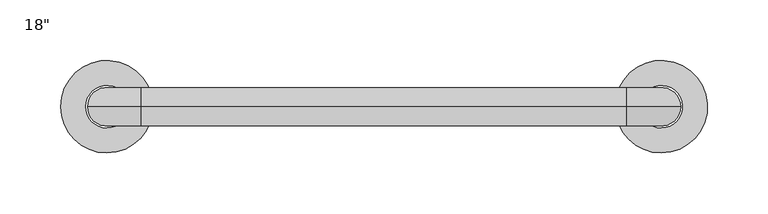
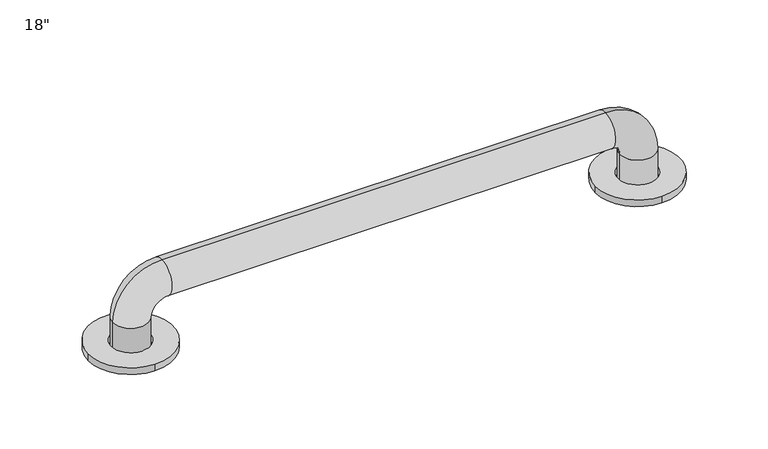
"""IFC4 building model written with IfcOpenShell, lengths in millimetres: proxy geometry."""

import ifcopenshell
import ifcopenshell.guid

model = None  # the IFC model being written
_history = None  # IfcOwnerHistory: only IFC2X3 demands one
_inside = {}  # id of a spatial element -> (the spatial element, [elements in it])
_under = {}  # id of a project, library or spatial element -> (it, [spatial elements below it])
_declared = {}  # id of a project -> (the project, [libraries it declares])
_typed = {}  # id of a type object -> (the type object, [elements of that type])
_made_of = {}  # id of a material, layer set ... -> (it, [elements and type objects made of it])


def new_model(schema):
    """Start an empty IFC model of exactly this schema.

    Asked for "IFC4X3", IfcOpenShell would pick the latest addendum, in which some entities
    have other attributes; the version numbers below select the first issue.
    IFC2X3 requires an IfcOwnerHistory on every rooted entity: one is made here for all.
    """
    global model, _history
    if schema == "IFC4X3":
        model = ifcopenshell.file(schema_version=(4, 3, 0, 0))
    else:
        model = ifcopenshell.file(schema=schema)
    _inside.clear()
    _under.clear()
    _declared.clear()
    _typed.clear()
    _made_of.clear()
    _history = None
    if model.schema == "IFC2X3":
        org = make("IfcOrganization", Name="unknown")
        user = make(
            "IfcPersonAndOrganization",
            ThePerson=make("IfcPerson", FamilyName="unknown"),
            TheOrganization=org,
        )
        app = make(
            "IfcApplication",
            ApplicationDeveloper=org,
            Version="unknown",
            ApplicationFullName="unknown",
            ApplicationIdentifier="unknown",
        )
        _history = make(
            "IfcOwnerHistory",
            OwningUser=user,
            OwningApplication=app,
            ChangeAction="ADDED",
            CreationDate=0,
        )
    return model


def make(cls, **values):
    """One entity of the class cls with the attributes given. An attribute that is None is left unset."""
    return model.create_entity(
        cls, **{name: value for name, value in values.items() if value is not None}
    )


def rooted(cls, **values):
    """An entity with a GlobalId (a new one), such as an element, a storey or a relation."""
    return make(cls, GlobalId=ifcopenshell.guid.new(), OwnerHistory=_history, **values)


def si_unit(unit_type, name, prefix=None):
    """IfcSIUnit, for example si_unit("LENGTHUNIT", "METRE", prefix="MILLI")."""
    return make("IfcSIUnit", UnitType=unit_type, Prefix=prefix, Name=name)


def assignment(units):
    """IfcUnitAssignment: the units of a project."""
    return None if units is None else make("IfcUnitAssignment", Units=units)


def point(xyz):
    """IfcCartesianPoint."""
    return None if xyz is None else make("IfcCartesianPoint", Coordinates=xyz)


def direction(xyz):
    """IfcDirection."""
    return None if xyz is None else make("IfcDirection", DirectionRatios=xyz)


def frame(location, z_axis=None, x_axis=None):
    """IfcAxis2Placement3D, a coordinate frame: its origin and axes. An axis left out is left unset."""
    return make(
        "IfcAxis2Placement3D",
        Location=point(location),
        Axis=direction(z_axis),
        RefDirection=direction(x_axis),
    )


def frame_2d(location, x_axis=None):
    """IfcAxis2Placement2D, a coordinate frame in the plane: its origin and x axis."""
    return make(
        "IfcAxis2Placement2D", Location=point(location), RefDirection=direction(x_axis)
    )


def origin():
    """The frame at (0, 0, 0) with its axes left unset."""
    return frame((0.0, 0.0, 0.0))


def origin_with_axes():
    """The frame at (0, 0, 0) with the z axis (0, 0, 1) and the x axis (1, 0, 0) written out."""
    return frame((0.0, 0.0, 0.0), z_axis=(0.0, 0.0, 1.0), x_axis=(1.0, 0.0, 0.0))


def origin_2d():
    """The frame at (0, 0) in the plane with its x axis left unset."""
    return frame_2d((0.0, 0.0))


def place(relative_to, where):
    """IfcLocalPlacement: puts the frame where relative to a parent placement (None: the world)."""
    return make(
        "IfcLocalPlacement", PlacementRelTo=relative_to, RelativePlacement=where
    )


def context(
    kind, dimensions, precision=None, world=None, true_north=None, identifier=None
):
    """IfcGeometricRepresentationContext, for example the 3D "Model" context."""
    return make(
        "IfcGeometricRepresentationContext",
        ContextIdentifier=identifier,
        ContextType=kind,
        CoordinateSpaceDimension=dimensions,
        Precision=precision,
        WorldCoordinateSystem=world,
        TrueNorth=true_north,
    )


def project(units=None, contexts=None):
    """IfcProject with its units and contexts."""
    return rooted(
        "IfcProject",
        Name="project",
        RepresentationContexts=contexts,
        UnitsInContext=assignment(units),
    )


def spatial(cls, under=None, at=None, **own):
    """A site, building, storey or space (cls), placed at a placement, below another one or the project."""
    s = rooted(cls, ObjectPlacement=at, **own)
    if under is not None:
        _under.setdefault(under.id(), (under, []))[1].append(s)
    return s


def circle_curve(where, radius):
    """IfcCircle in the frame where."""
    return make("IfcCircle", Position=where, Radius=radius)


def ellipse_curve(where, semi_axis1, semi_axis2):
    """IfcEllipse in the frame where."""
    return make(
        "IfcEllipse", Position=where, SemiAxis1=semi_axis1, SemiAxis2=semi_axis2
    )


def trimmed(basis, trim1, trim2, sense, master):
    """IfcTrimmedCurve: the piece of a basis curve between two trims."""
    return make(
        "IfcTrimmedCurve",
        BasisCurve=basis,
        Trim1=trim1,
        Trim2=trim2,
        SenseAgreement=sense,
        MasterRepresentation=master,
    )


def segment(curve, same_sense, transition):
    """IfcCompositeCurveSegment."""
    return make(
        "IfcCompositeCurveSegment",
        Transition=transition,
        SameSense=same_sense,
        ParentCurve=curve,
    )


def composite_curve(segments, self_intersect=None):
    """IfcCompositeCurve: segments joined end to end."""
    return make("IfcCompositeCurve", Segments=segments, SelfIntersect=self_intersect)


def outline(outer, holes=None, kind="AREA"):
    """IfcArbitraryClosedProfileDef: a profile drawn as a closed curve; with holes, ...WithVoids."""
    if holes is None:
        return make("IfcArbitraryClosedProfileDef", ProfileType=kind, OuterCurve=outer)
    return make(
        "IfcArbitraryProfileDefWithVoids",
        ProfileType=kind,
        OuterCurve=outer,
        InnerCurves=holes,
    )


def extrude(swept, where, along, depth):
    """IfcExtrudedAreaSolid: the profile swept, set in the frame where, extruded along a direction by depth."""
    return make(
        "IfcExtrudedAreaSolid",
        SweptArea=swept,
        Position=where,
        ExtrudedDirection=direction(along),
        Depth=depth,
    )


def shape(context_of_items, identifier, shape_type, items):
    """IfcShapeRepresentation: the items that make up one representation, for example the "Body"."""
    return make(
        "IfcShapeRepresentation",
        ContextOfItems=context_of_items,
        RepresentationIdentifier=identifier,
        RepresentationType=shape_type,
        Items=items,
    )


def source(mapping_origin, context_of_items, identifier, shape_type, items):
    """IfcRepresentationMap: a shape defined once, which mapped items show again and again."""
    return make(
        "IfcRepresentationMap",
        MappingOrigin=mapping_origin,
        MappedRepresentation=shape(context_of_items, identifier, shape_type, items),
    )


def transform(
    local_origin,
    x_axis=None,
    y_axis=None,
    z_axis=None,
    scale=None,
    scale2=None,
    scale3=None,
    uniform=True,
):
    """IfcCartesianTransformationOperator3D, or its non-uniform kind. x_axis, y_axis, z_axis: its Axis1, 2, 3."""
    if uniform:
        return make(
            "IfcCartesianTransformationOperator3D",
            Axis1=direction(x_axis),
            Axis2=direction(y_axis),
            LocalOrigin=point(local_origin),
            Scale=scale,
            Axis3=direction(z_axis),
        )
    return make(
        "IfcCartesianTransformationOperator3DnonUniform",
        Axis1=direction(x_axis),
        Axis2=direction(y_axis),
        LocalOrigin=point(local_origin),
        Scale=scale,
        Axis3=direction(z_axis),
        Scale2=scale2,
        Scale3=scale3,
    )


def mapped(mapping_source, mapping_target):
    """IfcMappedItem: shows the shape of a source again, moved by a transform."""
    return make(
        "IfcMappedItem", MappingSource=mapping_source, MappingTarget=mapping_target
    )


def made_of(thing, what):
    """Note that an element or type object is made of a material, layer set ...; save() writes the relation."""
    if what is not None:
        _made_of.setdefault(what.id(), (what, []))[1].append(thing)
    return thing


def element(
    cls,
    number,
    at=None,
    inside=None,
    cuts=None,
    type_object=None,
    material=None,
    context=None,
    identifier="Body",
    shape_type=None,
    held_by="IfcProductDefinitionShape",
    body=None,
    shapes=None,
    **own,
):
    """One element of the class cls, such as IfcWall. Its Tag is "e" and its number.

    at: its placement. inside: the storey or other place that contains it. cuts: it is an
    opening in that element (IfcRelVoidsElement). A single representation is given by context,
    identifier, shape_type and body (its items); several are given by shapes. held_by: the class
    of the entity that holds the representations. save() writes the other relations.
    """
    e = rooted(cls, Tag="e%d" % number, ObjectPlacement=at, **own)
    if body is not None:
        shapes = [shape(context, identifier, shape_type, body)]
    if shapes is not None:
        e.Representation = make(held_by, Representations=shapes)
    if inside is not None:
        _inside.setdefault(inside.id(), (inside, []))[1].append(e)
    if cuts is not None:
        rooted(
            "IfcRelVoidsElement", RelatingBuildingElement=cuts, RelatedOpeningElement=e
        )
    if type_object is not None:
        _typed.setdefault(type_object.id(), (type_object, []))[1].append(e)
    return made_of(e, material)


def aggregate(whole, parts):
    """IfcRelAggregates: a whole, such as a stair, and the parts it consists of."""
    return rooted("IfcRelAggregates", RelatingObject=whole, RelatedObjects=parts)


def save(model, path):
    """Write the relations noted so far, then the file.

    IfcRelAggregates (storeys below a building ...), IfcRelContainedInSpatialStructure (elements
    in a storey), IfcRelDefinesByType, IfcRelAssociatesMaterial and IfcRelDeclares: one each for
    every whole, place, type object, material and project.
    """
    for whole, parts in _under.values():
        aggregate(whole, parts)
    for where, things in _inside.values():
        rooted(
            "IfcRelContainedInSpatialStructure",
            RelatedElements=things,
            RelatingStructure=where,
        )
    for kind, things in _typed.values():
        rooted("IfcRelDefinesByType", RelatedObjects=things, RelatingType=kind)
    for what, things in _made_of.values():
        rooted("IfcRelAssociatesMaterial", RelatedObjects=things, RelatingMaterial=what)
    for by, libraries in _declared.values():
        rooted("IfcRelDeclares", RelatingContext=by, RelatedDefinitions=libraries)
    model.write(path)


def plane_surface(at):
    """IfcPlane: the flat surface through the origin of the frame at, square to its z axis."""
    return make("IfcPlane", Position=at)


def cylinder_surface(at, radius):
    """IfcCylindricalSurface: all points at the distance radius from the z axis of the frame at."""
    return make("IfcCylindricalSurface", Position=at, Radius=radius)


def revolved_surface(curve, axis_point, axis_direction):
    """IfcSurfaceOfRevolution: the curve turned about the line through axis_point along axis_direction."""
    return make(
        "IfcSurfaceOfRevolution",
        SweptCurve=make("IfcArbitraryOpenProfileDef", ProfileType="CURVE", Curve=curve),
        AxisPosition=make("IfcAxis1Placement", Location=point(axis_point), Axis=direction(axis_direction)),
    )


def advanced_brep(points, edges, surfaces, faces):
    """IfcAdvancedBrep: a solid bounded by faces that lie on surfaces and meet in shared edges.

    An edge is (start, end): straight between two places in points (the first is 0);
    or (start, end, curve); or (start, end, curve, False) where it runs against its curve.
    A face is (place in surfaces, loops), or (place, loops, False) where it looks against
    its surface's normal. A loop lists edges by number (the first is 1), with a minus sign
    where the edge is run from its end to its start. The first loop is the outer one.
    """
    corners = [point(p) for p in points]
    vertices = [make("IfcVertexPoint", VertexGeometry=c) for c in corners]
    made = []
    for start, end, *more in edges:
        made.append(
            make(
                "IfcEdgeCurve",
                EdgeStart=vertices[start],
                EdgeEnd=vertices[end],
                EdgeGeometry=more[0] if more else make("IfcPolyline", Points=[corners[start], corners[end]]),
                SameSense=more[1] if len(more) > 1 else True,
            )
        )
    hull = []
    for where, loops, *sense in faces:
        bounds = []
        for j, loop in enumerate(loops):
            ring = [make("IfcOrientedEdge", EdgeElement=made[abs(k) - 1], Orientation=k > 0) for k in loop]
            bounds.append(
                make(
                    "IfcFaceOuterBound" if j == 0 else "IfcFaceBound",
                    Bound=make("IfcEdgeLoop", EdgeList=ring),
                    Orientation=True,
                )
            )
        hull.append(make("IfcAdvancedFace", Bounds=bounds, FaceSurface=surfaces[where], SameSense=sense[0] if sense else True))
    return make("IfcAdvancedBrep", Outer=make("IfcClosedShell", CfsFaces=hull))


def proxy_9e031665(model_context):
    return source(origin(), model_context, "Body", "SolidModel", [
        extrude(outline(composite_curve([segment(trimmed(circle_curve(frame_2d((457.2, 0.0)), 38.1), [point((419.1, 0.0))], [point((457.2, -38.1))], False, "CARTESIAN"), True, "CONTINUOUS"), segment(trimmed(circle_curve(frame_2d((457.2, 0.0)), 38.1), [point((457.2, -38.1))], [point((419.1, 0.0))], False, "CARTESIAN"), True, "CONTINUOUS")], self_intersect=False), holes=[composite_curve([segment(trimmed(circle_curve(frame_2d((457.2, 0.0)), 17.4625), [point((439.7375, 0.0))], [point((457.2, -17.4625))], True, "CARTESIAN"), True, "CONTINUOUS"), segment(trimmed(circle_curve(frame_2d((457.2, 0.0)), 17.4625), [point((457.2, -17.4625))], [point((439.7375, 0.0))], True, "CARTESIAN"), True, "CONTINUOUS")], self_intersect=False)]), origin_with_axes(), (0.0, 0.0, 1.0), 6.35),
        extrude(outline(composite_curve([segment(trimmed(circle_curve(origin_2d(), 38.1), [point((-38.1, 0.0))], [point((0.0, -38.1))], False, "CARTESIAN"), True, "CONTINUOUS"), segment(trimmed(circle_curve(origin_2d(), 38.1), [point((0.0, -38.1))], [point((-38.1, 0.0))], False, "CARTESIAN"), True, "CONTINUOUS")], self_intersect=False), holes=[composite_curve([segment(trimmed(circle_curve(origin_2d(), 17.4625), [point((-17.4625, 0.0))], [point((0.0, -17.4625))], True, "CARTESIAN"), True, "CONTINUOUS"), segment(trimmed(circle_curve(origin_2d(), 17.4625), [point((0.0, -17.4625))], [point((-17.4625, 0.0))], True, "CARTESIAN"), True, "CONTINUOUS")], self_intersect=False)]), origin_with_axes(), (0.0, 0.0, 1.0), 6.35),
        advanced_brep(
        [(473.075, 0.0, 0.0), (441.325, 0.0, 0.0), (473.075, 0.0, 28.575), (441.325, 0.0, 28.575), (428.625, 0.0, 41.275), (428.625, 0.0, 73.025), (28.575, 0.0, 73.025), (28.575, 0.0, 41.275), (15.875, 0.0, 28.575), (-15.875, 0.0, 28.575), (-15.875, 0.0, 0.0), (15.875, 0.0, 0.0)],
        [
            (0, 1, circle_curve(frame((457.2, 0.0, 0.0), z_axis=(0.0, 0.0, -1.0), x_axis=(-1.0, 0.0, 0.0)), 15.875)),
            (1, 0, circle_curve(frame((457.2, 0.0, 0.0), z_axis=(0.0, 0.0, -1.0), x_axis=(-1.0, 0.0, 0.0)), 15.875)),
            (0, 2),
            (2, 3, circle_curve(frame((457.2, 0.0, 28.575), z_axis=(0.0, 0.0, -1.0), x_axis=(-1.0, 0.0, 0.0)), 15.875)),
            (3, 1),
            (3, 2, circle_curve(frame((457.2, 0.0, 28.575), z_axis=(0.0, 0.0, -1.0), x_axis=(-1.0, 0.0, 0.0)), 15.875)),
            (4, 3, circle_curve(frame((428.625, 0.0, 28.575), z_axis=(0.0, 1.0, 0.0), x_axis=(1.0, 0.0, 0.0)), 12.7)),
            (2, 5, circle_curve(frame((428.625, 0.0, 28.575), z_axis=(0.0, -1.0, 0.0), x_axis=(1.0, 0.0, 0.0)), 44.45)),
            (5, 4, circle_curve(frame((428.625, 0.0, 57.15), z_axis=(1.0, 0.0, 0.0), x_axis=(0.0, 0.0, -1.0)), 15.875)),
            (4, 5, circle_curve(frame((428.625, 0.0, 57.15), z_axis=(1.0, 0.0, 0.0), x_axis=(0.0, 0.0, -1.0)), 15.875)),
            (5, 6),
            (6, 7, circle_curve(frame((28.575, 0.0, 57.15), z_axis=(1.0, 0.0, 0.0), x_axis=(0.0, 0.0, -1.0)), 15.875)),
            (7, 4),
            (7, 6, circle_curve(frame((28.575, 0.0, 57.15), z_axis=(1.0, 0.0, 0.0), x_axis=(0.0, 0.0, -1.0)), 15.875)),
            (8, 7, circle_curve(frame((28.575, 0.0, 28.575), z_axis=(0.0, 1.0, 0.0), x_axis=(0.0, 0.0, 1.0)), 12.7)),
            (6, 9, circle_curve(frame((28.575, 0.0, 28.575), z_axis=(0.0, -1.0, 0.0), x_axis=(0.0, 0.0, 1.0)), 44.45)),
            (9, 8, circle_curve(frame((0.0, 0.0, 28.575), z_axis=(0.0, 0.0, 1.0), x_axis=(1.0, 0.0, 0.0)), 15.875)),
            (8, 9, circle_curve(frame((0.0, 0.0, 28.575), z_axis=(0.0, 0.0, 1.0), x_axis=(1.0, 0.0, 0.0)), 15.875)),
            (10, 11, circle_curve(frame((0.0, 0.0, 0.0), z_axis=(0.0, 0.0, -1.0), x_axis=(1.0, 0.0, 0.0)), 15.875)),
            (11, 10, circle_curve(frame((0.0, 0.0, 0.0), z_axis=(0.0, 0.0, -1.0), x_axis=(1.0, 0.0, 0.0)), 15.875)),
            (9, 10),
            (11, 8),
        ],
        [
            plane_surface(frame((457.2, 0.0, 0.0), z_axis=(0.0, 0.0, -1.0), x_axis=(0.0, -1.0, 0.0))),
            cylinder_surface(frame((457.2, 0.0, 0.0), z_axis=(0.0, 0.0, -1.0), x_axis=(-1.0, 0.0, 0.0)), 15.875),
            revolved_surface(trimmed(ellipse_curve(frame((457.2, 0.0, 28.575), z_axis=(0.0, 0.0, -1.0), x_axis=(-1.0, 0.0, 0.0)), 15.875, 15.875), [point((473.075, 0.0, 28.575))], [point((441.325, 0.0, 28.575))], True, "CARTESIAN"), (428.625, 0.0, 28.575), (0.0, -1.0, 0.0)),
            revolved_surface(trimmed(ellipse_curve(frame((457.2, 0.0, 28.575), z_axis=(0.0, 0.0, -1.0), x_axis=(-1.0, 0.0, 0.0)), 15.875, 15.875), [point((441.325, 0.0, 28.575))], [point((473.075, 0.0, 28.575))], True, "CARTESIAN"), (428.625, 0.0, 28.575), (0.0, -1.0, 0.0)),
            cylinder_surface(frame((428.625, 0.0, 57.15), z_axis=(1.0, 0.0, 0.0), x_axis=(0.0, 0.0, -1.0)), 15.875),
            revolved_surface(trimmed(ellipse_curve(frame((28.575, 0.0, 57.15), z_axis=(1.0, 0.0, 0.0), x_axis=(0.0, 0.0, -1.0)), 15.875, 15.875), [point((28.575, 0.0, 73.025))], [point((28.575, 0.0, 41.275))], True, "CARTESIAN"), (28.575, 0.0, 28.575), (0.0, -1.0, 0.0)),
            revolved_surface(trimmed(ellipse_curve(frame((28.575, 0.0, 57.15), z_axis=(1.0, 0.0, 0.0), x_axis=(0.0, 0.0, -1.0)), 15.875, 15.875), [point((28.575, 0.0, 41.275))], [point((28.575, 0.0, 73.025))], True, "CARTESIAN"), (28.575, 0.0, 28.575), (0.0, -1.0, 0.0)),
            plane_surface(frame((0.0, 0.0, 0.0), z_axis=(0.0, 0.0, -1.0), x_axis=(0.0, -1.0, 0.0))),
            cylinder_surface(frame((0.0, 0.0, 28.575), z_axis=(0.0, 0.0, 1.0), x_axis=(1.0, 0.0, 0.0)), 15.875),
        ],
        [
            (0, [[1, 2]]),
            (1, [[-1, 3, 4, 5]]),
            (1, [[-2, -5, 6, -3]]),
            (2, [[7, -4, 8, 9]]),
            (3, [[-8, -6, -7, 10]]),
            (4, [[-9, 11, 12, 13]]),
            (4, [[-10, -13, 14, -11]]),
            (5, [[15, -12, 16, 17]]),
            (6, [[-16, -14, -15, 18]]),
            (7, [[19, 20]]),
            (8, [[-17, 21, -20, 22]]),
            (8, [[-18, -22, -19, -21]]),
        ],
    ),
    ])


if __name__ == "__main__":
    model = new_model("IFC4")
    model_context = context("Model", 3, world=origin())
    ifc_project = project(units=[si_unit("LENGTHUNIT", "METRE", prefix="MILLI")], contexts=[model_context])
    site = spatial("IfcSite", under=ifc_project)
    building = spatial("IfcBuilding", under=site)
    placement = place(None, origin())
    proxy_shape = proxy_9e031665(model_context)
    element("IfcBuildingElementProxy", 1, Name="Seqm-Grab Bar : 18\"", ObjectType="Seqm-Grab Bar : 18\"", at=placement, inside=building, context=model_context, shape_type="MappedRepresentation", body=[
        mapped(proxy_shape, transform((0.0, 0.0, 0.0), x_axis=(1.0, 0.0, 0.0), y_axis=(0.0, 1.0, 0.0), z_axis=(0.0, 0.0, 1.0))),
    ])
    save(model, "model.ifc")

# Revit data of these elements
# Type "Seqm-Grab Bar : 18\""
#   Spec Number = "10 28 00"
#   Spec Description = "18\" GRAB BAR"
#   Length = 1' - 6"
#   Default Elevation = 4' - 0"
#   Grab Bar Material = GRAB BARS - AT ADA RESTROOMS ONLY
# Element 1 (IfcBuildingElementProxy, "Seqm-Grab Bar : 18\"")
#   Materials on its faces: "GRAB BARS - AT ADA RESTROOMS ONLY"
# Materials
#   "GRAB BARS - AT ADA RESTROOMS ONLY": class "Generic", colour RGB 120 120 120, transparency 0, Cost = 0
